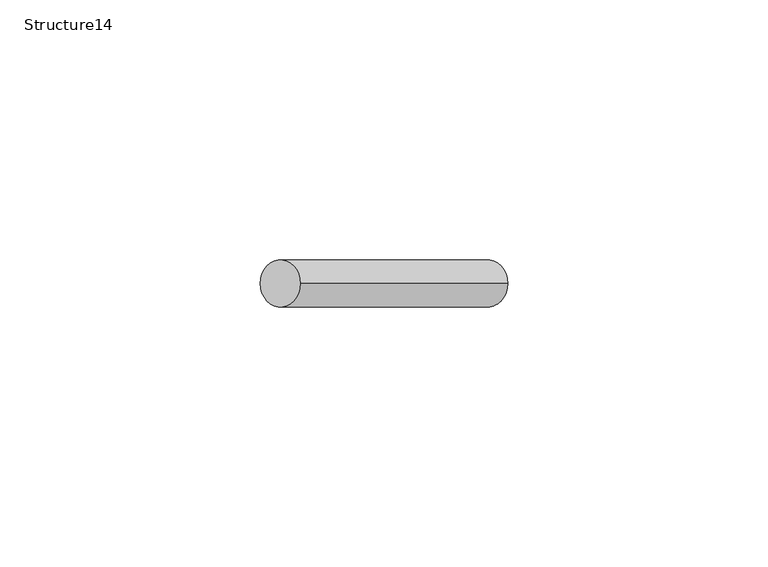
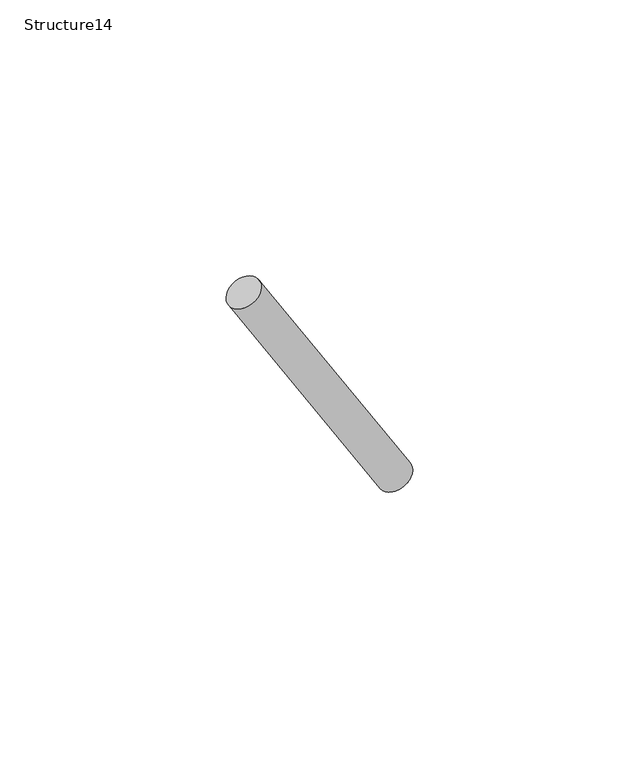
"""IFC4 building model written with IfcOpenShell, lengths in millimetres: proxy geometry, Structure14 : Structure668217135."""

from ifc_helpers import new_model, si_unit, point, frame, frame_2d, origin, place, context, project, spatial, circle_curve, trimmed, segment, composite_curve, outline, extrude, source, transform, mapped, element, save


def structure14_21772ca8(model_context):
    return source(origin(), model_context, "Body", "SweptSolid", [
        extrude(outline(composite_curve([segment(trimmed(circle_curve(frame_2d((0.0, -4.5217366)), 4.5217366), [point((0.0, -9.0434732))], [point((0.0, 0.0))], False, "CARTESIAN"), True, "CONTINUOUS"), segment(trimmed(circle_curve(frame_2d((0.0, -4.5217366)), 4.5217366), [point((0.0, 0.0))], [point((0.0, -9.0434732))], False, "CARTESIAN"), True, "CONTINUOUS")], self_intersect=False)), frame((7355.6151109, 1853.7780096, 39359.7840924), z_axis=(-0.523016219738758, 0.0, 0.8523227287185172), x_axis=(0.0, -1.0, 0.0)), (0.0, 0.0, 1.0), 76.2),
    ])


if __name__ == "__main__":
    model = new_model("IFC4")
    model_context = context("Model", 3, world=origin())
    ifc_project = project(units=[si_unit("LENGTHUNIT", "METRE", prefix="MILLI")], contexts=[model_context])
    site = spatial("IfcSite", under=ifc_project)
    building = spatial("IfcBuilding", under=site)
    placement = place(None, origin())
    structure14_shape = structure14_21772ca8(model_context)
    element("IfcBuildingElementProxy", 1, Name="Structure14 : Structure668217135", ObjectType="Structure14 : Structure668217135", at=placement, inside=building, context=model_context, shape_type="MappedRepresentation", body=[
        mapped(structure14_shape, transform((0.0, 0.0, 0.0), x_axis=(1.0, 0.0, 0.0), y_axis=(0.0, 1.0, 0.0), z_axis=(0.0, 0.0, 1.0))),
    ])
    save(model, "model.ifc")

# Revit data of these elements
# Type "Structure14 : Structure668217135"
#   NameOverride = "Structure668217135"
# Element 1 (IfcBuildingElementProxy, "Structure14 : Structure668217135")
#   Materials on its faces: "1.5\" DIA. STAINLESS STEEL RAILING"
# Materials
#   "1.5\" DIA. STAINLESS STEEL RAILING": class "Unassigned", colour RGB 128 128 128, transparency 0, Cost = 0
